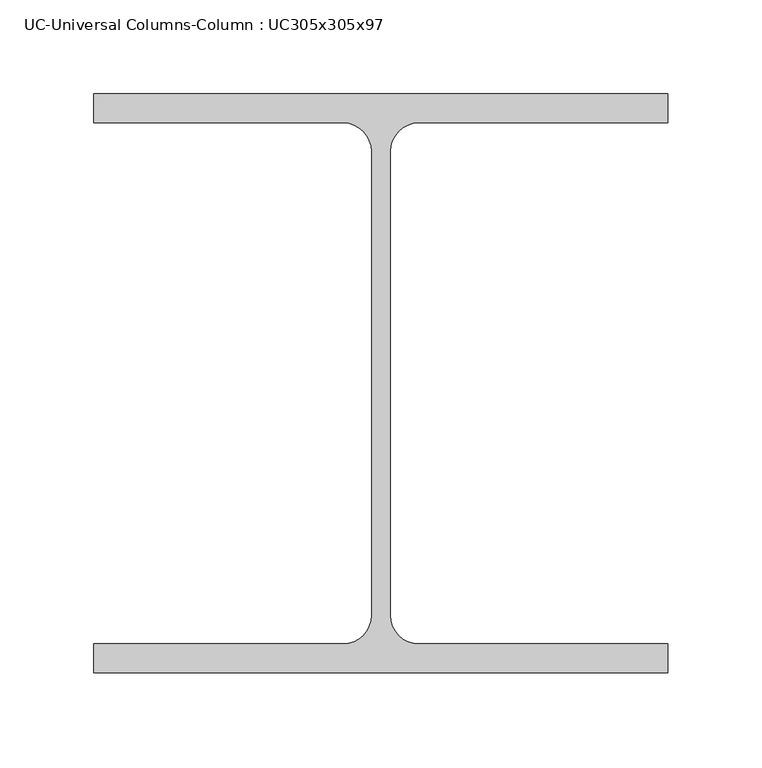
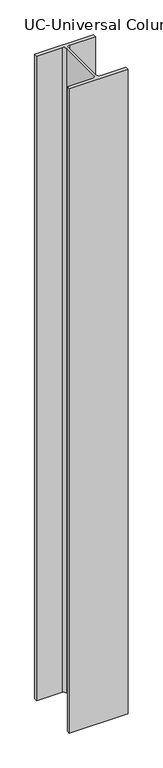
"""IFC4 building model written with IfcOpenShell, lengths in millimetres: column geometry, UC-Universal Columns-Column : UC305x305x97."""

from ifc_helpers import new_model, si_unit, point, frame_2d, origin, origin_with_axes, place, context, project, spatial, polyline, circle_curve, trimmed, segment, composite_curve, outline, extrude, source, transform, mapped, element, save


def uc_universal_columns_column_uc305x305x97_66ed23b3(model_context):
    return source(origin(), model_context, "Body", "SweptSolid", [
        extrude(outline(composite_curve([segment(polyline([(152.65, 153.95), (152.65, 138.55), (20.15, 138.55)]), True, "CONTINUOUS"), segment(trimmed(circle_curve(frame_2d((20.15, 123.35)), 15.2), [point((20.15, 138.55))], [point((4.95, 123.35))], True, "CARTESIAN"), True, "CONTINUOUS"), segment(polyline([(4.95, 123.35), (4.95, -123.35)]), True, "CONTINUOUS"), segment(trimmed(circle_curve(frame_2d((20.15, -123.35)), 15.2), [point((4.95, -123.35))], [point((20.15, -138.55))], True, "CARTESIAN"), True, "CONTINUOUS"), segment(polyline([(20.15, -138.55), (152.65, -138.55), (152.65, -153.95), (-152.65, -153.95), (-152.65, -138.55), (-20.15, -138.55)]), True, "CONTINUOUS"), segment(trimmed(circle_curve(frame_2d((-20.15, -123.35)), 15.2), [point((-20.15, -138.55))], [point((-4.95, -123.35))], True, "CARTESIAN"), True, "CONTINUOUS"), segment(polyline([(-4.95, -123.35), (-4.95, 123.35)]), True, "CONTINUOUS"), segment(trimmed(circle_curve(frame_2d((-20.15, 123.35)), 15.2), [point((-4.95, 123.35))], [point((-20.15, 138.55))], True, "CARTESIAN"), True, "CONTINUOUS"), segment(polyline([(-20.15, 138.55), (-152.65, 138.55), (-152.65, 153.95), (152.65, 153.95)]), True, "CONTINUOUS")], self_intersect=False)), origin_with_axes(), (0.0, 0.0, 1.0), 3530.0),
    ])


if __name__ == "__main__":
    model = new_model("IFC4")
    model_context = context("Model", 3, world=origin())
    ifc_project = project(units=[si_unit("LENGTHUNIT", "METRE", prefix="MILLI")], contexts=[model_context])
    site = spatial("IfcSite", under=ifc_project)
    building = spatial("IfcBuilding", under=site)
    placement = place(None, origin())
    uc_universal_columns_column_uc305x305x97_shape = uc_universal_columns_column_uc305x305x97_66ed23b3(model_context)
    element("IfcColumn", 1, ObjectType="UC-Universal Columns-Column : UC305x305x97", at=placement, inside=building, context=model_context, shape_type="MappedRepresentation", body=[
        mapped(uc_universal_columns_column_uc305x305x97_shape, transform((0.0, 0.0, 0.0), x_axis=(1.0, 0.0, 0.0), y_axis=(0.0, 1.0, 0.0), z_axis=(0.0, 0.0, 1.0))),
    ])
    save(model, "model.ifc")

# Revit data of these elements
# Type "UC-Universal Columns-Column : UC305x305x97"
#   Section Name Key = "UC305x305x97"
#   Width = 30.53 cm
#   Web Thickness = 0.99 cm
#   Web Fillet = 1.52 cm
#   Warping Constant = 1560000.0 cm⁶
#   Torsional Moment of Inertia = 91.20 cm⁴
#   Section Area = 123.0 cm²
#   Plastic Modulus weak axis = 726.0 cm³
#   Plastic Modulus strong axis = 1592.0 cm³
#   Nominal Weight = 96.8996 kgf/m
#   Moment of Inertia weak axis = 7308.00 cm⁴
#   Moment of Inertia strong axis = 22249.00 cm⁴
#   Height = 30.79 cm
#   Flange Thickness = 1.54 cm
#   Elastic Modulus weak axis = 479.0 cm³
#   Elastic Modulus strong axis = 1445.0 cm³
#   Centroid Vertical = 15.395 cm
#   Centroid Horizontal = 15.265 cm
#   Bolt Spacing = 14.0 cm
#   Structural Material [instance default] = Metal - Steel 43-275
#   Type Comments = ""
#   Assembly Code = ""
# Element 1 (IfcColumn, "UC-Universal Columns-Column : UC305x305x97")
#   Materials on its faces: "Metal - Steel 43-275"
# Materials
#   "Metal - Steel 43-275": class "Metal", colour RGB 247 247 247, transparency 0, Cost = 0
